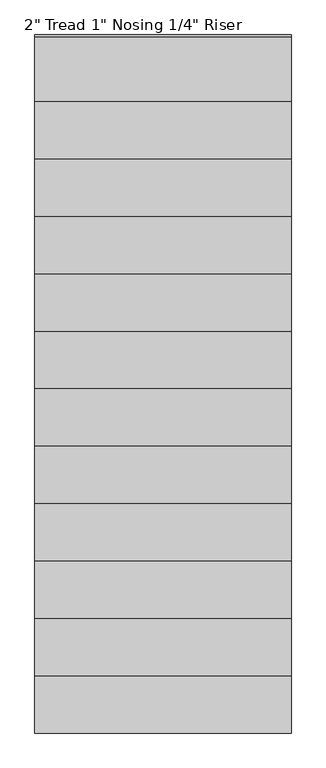
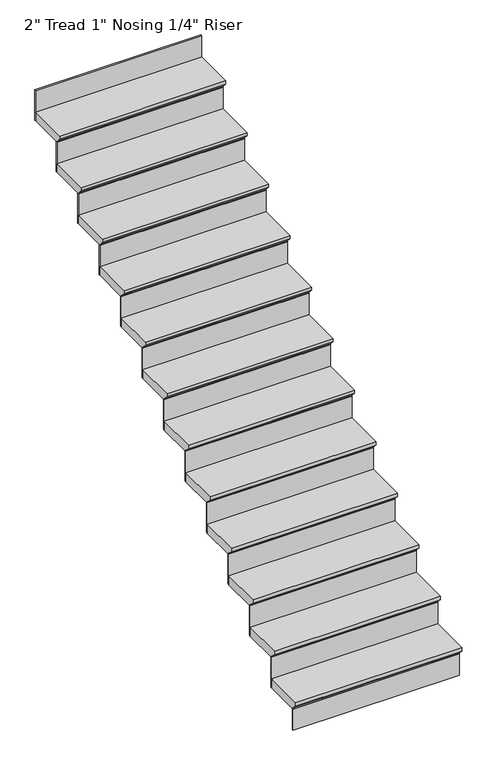
"""IFC4 building model written with IfcOpenShell, lengths in millimetres: stair flight geometry."""

from ifc_helpers import new_model, si_unit, frame, origin, place, context, project, spatial, polyline, outline, extrude, source, transform, mapped, element, save


def stair_flight_443dce11(model_context):
    return source(origin(), model_context, "Body", "SweptSolid", [
        extrude(outline(polyline([(-12572.2570712, -2092.5692308), (-12343.6570712, -2092.5692308), (-12343.6570712, -2143.3692308), (-12546.8570712, -2143.3692308), (-12546.8570712, -2137.0192308), (-12572.2570712, -2111.6192308), (-12572.2570712, -2092.5692308)])), frame((-25042.4664763, 0.0, 0.0), z_axis=(1.0, 0.0, 0.0), x_axis=(0.0, 1.0, 0.0)), (0.0, 0.0, 1.0), 908.05),
        extrude(outline(polyline([(-24134.4164763, -12540.5070712), (-24134.4164763, -12546.8570712), (-25042.4664763, -12546.8570712), (-25042.4664763, -12540.5070712), (-24134.4164763, -12540.5070712)])), frame((0.0, 0.0, -2266.95), z_axis=(0.0, 0.0, 1.0), x_axis=(1.0, 0.0, 0.0)), (0.0, 0.0, 1.0), 123.5807692),
        extrude(outline(polyline([(-24134.4164763, -12337.3070712), (-24134.4164763, -12343.6570712), (-25042.4664763, -12343.6570712), (-25042.4664763, -12337.3070712), (-24134.4164763, -12337.3070712)])), frame((0.0, 0.0, -2143.3692308), z_axis=(0.0, 0.0, 1.0), x_axis=(1.0, 0.0, 0.0)), (0.0, 0.0, 1.0), 174.3807692),
        extrude(outline(polyline([(-12369.0570712, -1918.1884615), (-12140.4570712, -1918.1884615), (-12140.4570712, -1968.9884615), (-12343.6570712, -1968.9884615), (-12343.6570712, -1962.6384615), (-12369.0570712, -1937.2384615), (-12369.0570712, -1918.1884615)])), frame((-25042.4664763, 0.0, 0.0), z_axis=(1.0, 0.0, 0.0), x_axis=(0.0, 1.0, 0.0)), (0.0, 0.0, 1.0), 908.05),
        extrude(outline(polyline([(-24134.4164763, -12134.1070712), (-24134.4164763, -12140.4570712), (-25042.4664763, -12140.4570712), (-25042.4664763, -12134.1070712), (-24134.4164763, -12134.1070712)])), frame((0.0, 0.0, -1968.9884615), z_axis=(0.0, 0.0, 1.0), x_axis=(1.0, 0.0, 0.0)), (0.0, 0.0, 1.0), 174.3807692),
        extrude(outline(polyline([(-12165.8570712, -1743.8076923), (-11937.2570712, -1743.8076923), (-11937.2570712, -1794.6076923), (-12140.4570712, -1794.6076923), (-12140.4570712, -1788.2576923), (-12165.8570712, -1762.8576923), (-12165.8570712, -1743.8076923)])), frame((-25042.4664763, 0.0, 0.0), z_axis=(1.0, 0.0, 0.0), x_axis=(0.0, 1.0, 0.0)), (0.0, 0.0, 1.0), 908.05),
        extrude(outline(polyline([(-24134.4164763, -11930.9070712), (-24134.4164763, -11937.2570712), (-25042.4664763, -11937.2570712), (-25042.4664763, -11930.9070712), (-24134.4164763, -11930.9070712)])), frame((0.0, 0.0, -1794.6076923), z_axis=(0.0, 0.0, 1.0), x_axis=(1.0, 0.0, 0.0)), (0.0, 0.0, 1.0), 174.3807692),
        extrude(outline(polyline([(-11962.6570712, -1569.4269231), (-11734.0570712, -1569.4269231), (-11734.0570712, -1620.2269231), (-11937.2570712, -1620.2269231), (-11937.2570712, -1613.8769231), (-11962.6570712, -1588.4769231), (-11962.6570712, -1569.4269231)])), frame((-25042.4664763, 0.0, 0.0), z_axis=(1.0, 0.0, 0.0), x_axis=(0.0, 1.0, 0.0)), (0.0, 0.0, 1.0), 908.05),
        extrude(outline(polyline([(-24134.4164763, -11727.7070712), (-24134.4164763, -11734.0570712), (-25042.4664763, -11734.0570712), (-25042.4664763, -11727.7070712), (-24134.4164763, -11727.7070712)])), frame((0.0, 0.0, -1620.2269231), z_axis=(0.0, 0.0, 1.0), x_axis=(1.0, 0.0, 0.0)), (0.0, 0.0, 1.0), 174.3807692),
        extrude(outline(polyline([(-11759.4570712, -1395.0461538), (-11530.8570712, -1395.0461538), (-11530.8570712, -1445.8461538), (-11734.0570712, -1445.8461538), (-11734.0570712, -1439.4961538), (-11759.4570712, -1414.0961538), (-11759.4570712, -1395.0461538)])), frame((-25042.4664763, 0.0, 0.0), z_axis=(1.0, 0.0, 0.0), x_axis=(0.0, 1.0, 0.0)), (0.0, 0.0, 1.0), 908.05),
        extrude(outline(polyline([(-24134.4164763, -11524.5070712), (-24134.4164763, -11530.8570712), (-25042.4664763, -11530.8570712), (-25042.4664763, -11524.5070712), (-24134.4164763, -11524.5070712)])), frame((0.0, 0.0, -1445.8461538), z_axis=(0.0, 0.0, 1.0), x_axis=(1.0, 0.0, 0.0)), (0.0, 0.0, 1.0), 174.3807692),
        extrude(outline(polyline([(-11556.2570712, -1220.6653846), (-11327.6570712, -1220.6653846), (-11327.6570712, -1271.4653846), (-11530.8570712, -1271.4653846), (-11530.8570712, -1265.1153846), (-11556.2570712, -1239.7153846), (-11556.2570712, -1220.6653846)])), frame((-25042.4664763, 0.0, 0.0), z_axis=(1.0, 0.0, 0.0), x_axis=(0.0, 1.0, 0.0)), (0.0, 0.0, 1.0), 908.05),
        extrude(outline(polyline([(-24134.4164763, -11321.3070712), (-24134.4164763, -11327.6570712), (-25042.4664763, -11327.6570712), (-25042.4664763, -11321.3070712), (-24134.4164763, -11321.3070712)])), frame((0.0, 0.0, -1271.4653846), z_axis=(0.0, 0.0, 1.0), x_axis=(1.0, 0.0, 0.0)), (0.0, 0.0, 1.0), 174.3807692),
        extrude(outline(polyline([(-11353.0570712, -1046.2846154), (-11124.4570712, -1046.2846154), (-11124.4570712, -1097.0846154), (-11327.6570712, -1097.0846154), (-11327.6570712, -1090.7346154), (-11353.0570712, -1065.3346154), (-11353.0570712, -1046.2846154)])), frame((-25042.4664763, 0.0, 0.0), z_axis=(1.0, 0.0, 0.0), x_axis=(0.0, 1.0, 0.0)), (0.0, 0.0, 1.0), 908.05),
        extrude(outline(polyline([(-24134.4164763, -11118.1070712), (-24134.4164763, -11124.4570712), (-25042.4664763, -11124.4570712), (-25042.4664763, -11118.1070712), (-24134.4164763, -11118.1070712)])), frame((0.0, 0.0, -1097.0846154), z_axis=(0.0, 0.0, 1.0), x_axis=(1.0, 0.0, 0.0)), (0.0, 0.0, 1.0), 174.3807692),
        extrude(outline(polyline([(-11149.8570712, -871.9038462), (-10921.2570712, -871.9038462), (-10921.2570712, -922.7038462), (-11124.4570712, -922.7038462), (-11124.4570712, -916.3538462), (-11149.8570712, -890.9538462), (-11149.8570712, -871.9038462)])), frame((-25042.4664763, 0.0, 0.0), z_axis=(1.0, 0.0, 0.0), x_axis=(0.0, 1.0, 0.0)), (0.0, 0.0, 1.0), 908.05),
        extrude(outline(polyline([(-24134.4164763, -10914.9070712), (-24134.4164763, -10921.2570712), (-25042.4664763, -10921.2570712), (-25042.4664763, -10914.9070712), (-24134.4164763, -10914.9070712)])), frame((0.0, 0.0, -922.7038462), z_axis=(0.0, 0.0, 1.0), x_axis=(1.0, 0.0, 0.0)), (0.0, 0.0, 1.0), 174.3807692),
        extrude(outline(polyline([(-10946.6570712, -697.5230769), (-10718.0570712, -697.5230769), (-10718.0570712, -748.3230769), (-10921.2570712, -748.3230769), (-10921.2570712, -741.9730769), (-10946.6570712, -716.5730769), (-10946.6570712, -697.5230769)])), frame((-25042.4664763, 0.0, 0.0), z_axis=(1.0, 0.0, 0.0), x_axis=(0.0, 1.0, 0.0)), (0.0, 0.0, 1.0), 908.05),
        extrude(outline(polyline([(-24134.4164763, -10711.7070712), (-24134.4164763, -10718.0570712), (-25042.4664763, -10718.0570712), (-25042.4664763, -10711.7070712), (-24134.4164763, -10711.7070712)])), frame((0.0, 0.0, -748.3230769), z_axis=(0.0, 0.0, 1.0), x_axis=(1.0, 0.0, 0.0)), (0.0, 0.0, 1.0), 174.3807692),
        extrude(outline(polyline([(-10743.4570712, -523.1423077), (-10514.8570712, -523.1423077), (-10514.8570712, -573.9423077), (-10718.0570712, -573.9423077), (-10718.0570712, -567.5923077), (-10743.4570712, -542.1923077), (-10743.4570712, -523.1423077)])), frame((-25042.4664763, 0.0, 0.0), z_axis=(1.0, 0.0, 0.0), x_axis=(0.0, 1.0, 0.0)), (0.0, 0.0, 1.0), 908.05),
        extrude(outline(polyline([(-24134.4164763, -10508.5070712), (-24134.4164763, -10514.8570712), (-25042.4664763, -10514.8570712), (-25042.4664763, -10508.5070712), (-24134.4164763, -10508.5070712)])), frame((0.0, 0.0, -573.9423077), z_axis=(0.0, 0.0, 1.0), x_axis=(1.0, 0.0, 0.0)), (0.0, 0.0, 1.0), 174.3807692),
        extrude(outline(polyline([(-10540.2570712, -348.7615385), (-10311.6570712, -348.7615385), (-10311.6570712, -399.5615385), (-10514.8570712, -399.5615385), (-10514.8570712, -393.2115385), (-10540.2570712, -367.8115385), (-10540.2570712, -348.7615385)])), frame((-25042.4664763, 0.0, 0.0), z_axis=(1.0, 0.0, 0.0), x_axis=(0.0, 1.0, 0.0)), (0.0, 0.0, 1.0), 908.05),
        extrude(outline(polyline([(-24134.4164763, -10305.3070712), (-24134.4164763, -10311.6570712), (-25042.4664763, -10311.6570712), (-25042.4664763, -10305.3070712), (-24134.4164763, -10305.3070712)])), frame((0.0, 0.0, -399.5615385), z_axis=(0.0, 0.0, 1.0), x_axis=(1.0, 0.0, 0.0)), (0.0, 0.0, 1.0), 174.3807692),
        extrude(outline(polyline([(-24134.4164763, -10102.1070712), (-24134.4164763, -10108.4570712), (-25042.4664763, -10108.4570712), (-25042.4664763, -10102.1070712), (-24134.4164763, -10102.1070712)])), frame((0.0, 0.0, -225.1807692), z_axis=(0.0, 0.0, 1.0), x_axis=(1.0, 0.0, 0.0)), (0.0, 0.0, 1.0), 174.3807692),
        extrude(outline(polyline([(-10337.0570712, -174.3807692), (-10108.4570712, -174.3807692), (-10108.4570712, -225.1807692), (-10311.6570712, -225.1807692), (-10311.6570712, -218.8307692), (-10337.0570712, -193.4307692), (-10337.0570712, -174.3807692)])), frame((-25042.4664763, 0.0, 0.0), z_axis=(1.0, 0.0, 0.0), x_axis=(0.0, 1.0, 0.0)), (0.0, 0.0, 1.0), 908.05),
    ])


if __name__ == "__main__":
    model = new_model("IFC4")
    model_context = context("Model", 3, world=origin())
    ifc_project = project(units=[si_unit("LENGTHUNIT", "METRE", prefix="MILLI")], contexts=[model_context])
    site = spatial("IfcSite", under=ifc_project)
    building = spatial("IfcBuilding", under=site)
    placement = place(None, origin())
    stair_flight_shape = stair_flight_443dce11(model_context)
    element("IfcStairFlight", 1, ObjectType="2\" Tread 1\" Nosing 1/4\" Riser", at=placement, inside=building, context=model_context, shape_type="MappedRepresentation", body=[
        mapped(stair_flight_shape, transform((0.0, 0.0, 0.0), x_axis=(1.0, 0.0, 0.0), y_axis=(0.0, 1.0, 0.0), z_axis=(0.0, 0.0, 1.0))),
    ])
    save(model, "model.ifc")
